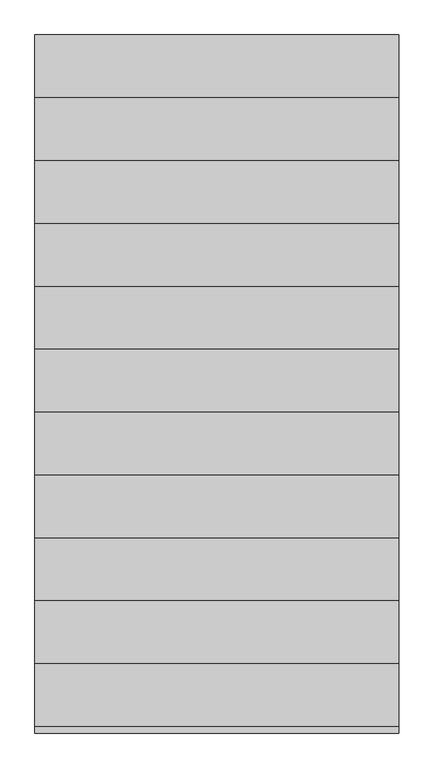
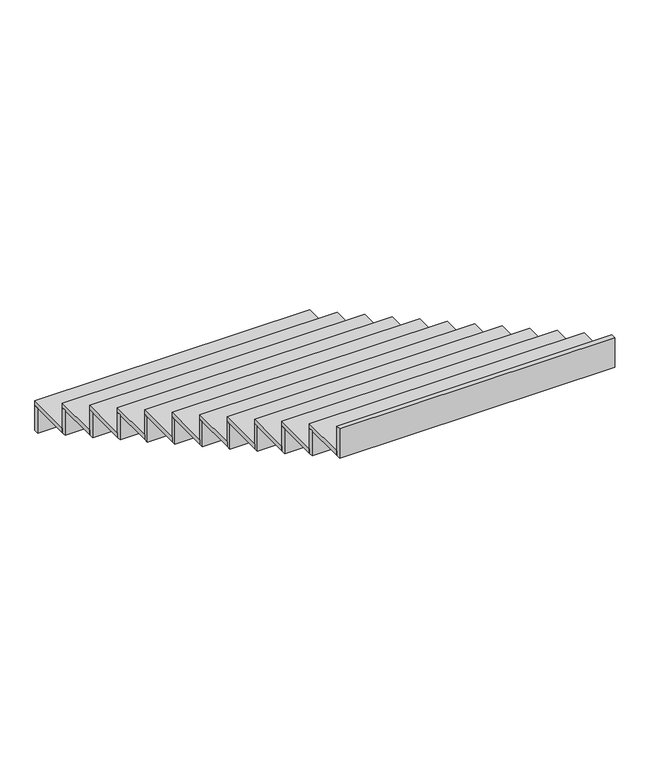
"""IFC4 building model written with IfcOpenShell, lengths in millimetres: stair flight geometry."""

from ifc_helpers import new_model, si_unit, frame, origin, place, context, project, spatial, polyline, outline, extrude, source, transform, mapped, element, save


def stair_flight_ce757a3a(model_context):
    return source(origin(), model_context, "Body", "SweptSolid", [
        extrude(outline(polyline([(52915.0, -2330.0), (52915.0, -2300.0), (54650.0, -2300.0), (54650.0, -2330.0), (52915.0, -2330.0)])), frame((0.0, 0.0, 14770.0), z_axis=(0.0, 0.0, 1.0), x_axis=(1.0, 0.0, 0.0)), (0.0, 0.0, 1.0), 166.6666667),
        extrude(outline(polyline([(54650.0, -2600.0), (52915.0, -2600.0), (52915.0, -2300.0), (54650.0, -2300.0), (54650.0, -2600.0)])), frame((0.0, 0.0, 14936.6666667), z_axis=(0.0, 0.0, 1.0), x_axis=(1.0, 0.0, 0.0)), (0.0, 0.0, 1.0), 30.0),
        extrude(outline(polyline([(52915.0, -2630.0), (52915.0, -2600.0), (54650.0, -2600.0), (54650.0, -2630.0), (52915.0, -2630.0)])), frame((0.0, 0.0, 14936.6666667), z_axis=(0.0, 0.0, 1.0), x_axis=(1.0, 0.0, 0.0)), (0.0, 0.0, 1.0), 166.6666667),
        extrude(outline(polyline([(54650.0, -2900.0), (52915.0, -2900.0), (52915.0, -2600.0), (54650.0, -2600.0), (54650.0, -2900.0)])), frame((0.0, 0.0, 15103.3333333), z_axis=(0.0, 0.0, 1.0), x_axis=(1.0, 0.0, 0.0)), (0.0, 0.0, 1.0), 30.0),
        extrude(outline(polyline([(52915.0, -2930.0), (52915.0, -2900.0), (54650.0, -2900.0), (54650.0, -2930.0), (52915.0, -2930.0)])), frame((0.0, 0.0, 15103.3333333), z_axis=(0.0, 0.0, 1.0), x_axis=(1.0, 0.0, 0.0)), (0.0, 0.0, 1.0), 166.6666667),
        extrude(outline(polyline([(54650.0, -3200.0), (52915.0, -3200.0), (52915.0, -2900.0), (54650.0, -2900.0), (54650.0, -3200.0)])), frame((0.0, 0.0, 15270.0), z_axis=(0.0, 0.0, 1.0), x_axis=(1.0, 0.0, 0.0)), (0.0, 0.0, 1.0), 30.0),
        extrude(outline(polyline([(52915.0, -3230.0), (52915.0, -3200.0), (54650.0, -3200.0), (54650.0, -3230.0), (52915.0, -3230.0)])), frame((0.0, 0.0, 15270.0), z_axis=(0.0, 0.0, 1.0), x_axis=(1.0, 0.0, 0.0)), (0.0, 0.0, 1.0), 166.6666667),
        extrude(outline(polyline([(54650.0, -3500.0), (52915.0, -3500.0), (52915.0, -3200.0), (54650.0, -3200.0), (54650.0, -3500.0)])), frame((0.0, 0.0, 15436.6666667), z_axis=(0.0, 0.0, 1.0), x_axis=(1.0, 0.0, 0.0)), (0.0, 0.0, 1.0), 30.0),
        extrude(outline(polyline([(52915.0, -3530.0), (52915.0, -3500.0), (54650.0, -3500.0), (54650.0, -3530.0), (52915.0, -3530.0)])), frame((0.0, 0.0, 15436.6666667), z_axis=(0.0, 0.0, 1.0), x_axis=(1.0, 0.0, 0.0)), (0.0, 0.0, 1.0), 166.6666667),
        extrude(outline(polyline([(54650.0, -3800.0), (52915.0, -3800.0), (52915.0, -3500.0), (54650.0, -3500.0), (54650.0, -3800.0)])), frame((0.0, 0.0, 15603.3333333), z_axis=(0.0, 0.0, 1.0), x_axis=(1.0, 0.0, 0.0)), (0.0, 0.0, 1.0), 30.0),
        extrude(outline(polyline([(52915.0, -3830.0), (52915.0, -3800.0), (54650.0, -3800.0), (54650.0, -3830.0), (52915.0, -3830.0)])), frame((0.0, 0.0, 15603.3333333), z_axis=(0.0, 0.0, 1.0), x_axis=(1.0, 0.0, 0.0)), (0.0, 0.0, 1.0), 166.6666667),
        extrude(outline(polyline([(54650.0, -4100.0), (52915.0, -4100.0), (52915.0, -3800.0), (54650.0, -3800.0), (54650.0, -4100.0)])), frame((0.0, 0.0, 15770.0), z_axis=(0.0, 0.0, 1.0), x_axis=(1.0, 0.0, 0.0)), (0.0, 0.0, 1.0), 30.0),
        extrude(outline(polyline([(52915.0, -4130.0), (52915.0, -4100.0), (54650.0, -4100.0), (54650.0, -4130.0), (52915.0, -4130.0)])), frame((0.0, 0.0, 15770.0), z_axis=(0.0, 0.0, 1.0), x_axis=(1.0, 0.0, 0.0)), (0.0, 0.0, 1.0), 166.6666667),
        extrude(outline(polyline([(54650.0, -4400.0), (52915.0, -4400.0), (52915.0, -4100.0), (54650.0, -4100.0), (54650.0, -4400.0)])), frame((0.0, 0.0, 15936.6666667), z_axis=(0.0, 0.0, 1.0), x_axis=(1.0, 0.0, 0.0)), (0.0, 0.0, 1.0), 30.0),
        extrude(outline(polyline([(52915.0, -4430.0), (52915.0, -4400.0), (54650.0, -4400.0), (54650.0, -4430.0), (52915.0, -4430.0)])), frame((0.0, 0.0, 15936.6666667), z_axis=(0.0, 0.0, 1.0), x_axis=(1.0, 0.0, 0.0)), (0.0, 0.0, 1.0), 166.6666667),
        extrude(outline(polyline([(54650.0, -4700.0), (52915.0, -4700.0), (52915.0, -4400.0), (54650.0, -4400.0), (54650.0, -4700.0)])), frame((0.0, 0.0, 16103.3333333), z_axis=(0.0, 0.0, 1.0), x_axis=(1.0, 0.0, 0.0)), (0.0, 0.0, 1.0), 30.0),
        extrude(outline(polyline([(52915.0, -4730.0), (52915.0, -4700.0), (54650.0, -4700.0), (54650.0, -4730.0), (52915.0, -4730.0)])), frame((0.0, 0.0, 16103.3333333), z_axis=(0.0, 0.0, 1.0), x_axis=(1.0, 0.0, 0.0)), (0.0, 0.0, 1.0), 166.6666667),
        extrude(outline(polyline([(54650.0, -5000.0), (52915.0, -5000.0), (52915.0, -4700.0), (54650.0, -4700.0), (54650.0, -5000.0)])), frame((0.0, 0.0, 16270.0), z_axis=(0.0, 0.0, 1.0), x_axis=(1.0, 0.0, 0.0)), (0.0, 0.0, 1.0), 30.0),
        extrude(outline(polyline([(52915.0, -5030.0), (52915.0, -5000.0), (54650.0, -5000.0), (54650.0, -5030.0), (52915.0, -5030.0)])), frame((0.0, 0.0, 16270.0), z_axis=(0.0, 0.0, 1.0), x_axis=(1.0, 0.0, 0.0)), (0.0, 0.0, 1.0), 166.6666667),
        extrude(outline(polyline([(54650.0, -5300.0), (52915.0, -5300.0), (52915.0, -5000.0), (54650.0, -5000.0), (54650.0, -5300.0)])), frame((0.0, 0.0, 16436.6666667), z_axis=(0.0, 0.0, 1.0), x_axis=(1.0, 0.0, 0.0)), (0.0, 0.0, 1.0), 30.0),
        extrude(outline(polyline([(52915.0, -5330.0), (52915.0, -5300.0), (54650.0, -5300.0), (54650.0, -5330.0), (52915.0, -5330.0)])), frame((0.0, 0.0, 16436.6666667), z_axis=(0.0, 0.0, 1.0), x_axis=(1.0, 0.0, 0.0)), (0.0, 0.0, 1.0), 166.6666667),
        extrude(outline(polyline([(52915.0, -5630.0), (52915.0, -5600.0), (54650.0, -5600.0), (54650.0, -5630.0), (52915.0, -5630.0)])), frame((0.0, 0.0, 16603.3333333), z_axis=(0.0, 0.0, 1.0), x_axis=(1.0, 0.0, 0.0)), (0.0, 0.0, 1.0), 196.6666667),
        extrude(outline(polyline([(54650.0, -5600.0), (52915.0, -5600.0), (52915.0, -5300.0), (54650.0, -5300.0), (54650.0, -5600.0)])), frame((0.0, 0.0, 16603.3333333), z_axis=(0.0, 0.0, 1.0), x_axis=(1.0, 0.0, 0.0)), (0.0, 0.0, 1.0), 30.0),
    ])


if __name__ == "__main__":
    model = new_model("IFC4")
    model_context = context("Model", 3, world=origin())
    ifc_project = project(units=[si_unit("LENGTHUNIT", "METRE", prefix="MILLI")], contexts=[model_context])
    site = spatial("IfcSite", under=ifc_project)
    building = spatial("IfcBuilding", under=site)
    placement = place(None, origin())
    stair_flight_shape = stair_flight_ce757a3a(model_context)
    element("IfcStairFlight", 1, at=placement, inside=building, context=model_context, shape_type="MappedRepresentation", body=[
        mapped(stair_flight_shape, transform((0.0, 0.0, 0.0), x_axis=(1.0, 0.0, 0.0), y_axis=(0.0, 1.0, 0.0), z_axis=(0.0, 0.0, 1.0))),
    ])
    save(model, "model.ifc")

# Revit data of these elements
# Element 1 (IfcStairFlight)
#   Materials on its faces: "00_Finish_Deco Tile"
# Materials
#   "00_Finish_Deco Tile": class "Finish", colour RGB 245 245 245, transparency 0, Description = "Ceramic Tile", Cost = 0
